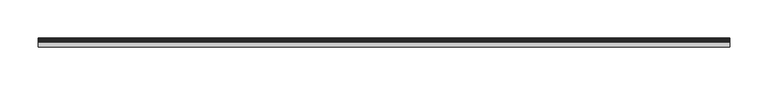
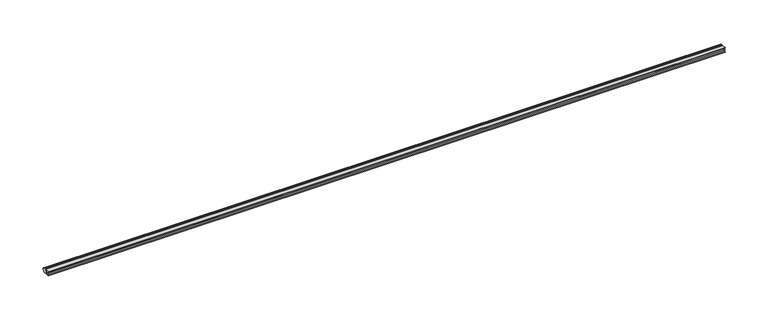
"""IFC4 building model written with IfcOpenShell, lengths in millimetres: proxy geometry, Generic Models 7:Generic Models 1:1:Generic Models 1:1 : Generic Models 7:Generic Models 1:337419:44 : Generic Models 7:Generic Models 1:1:Generic Models 1:1 : Generic Models 7:Generic Models 1:337419:306201."""

from ifc_helpers import new_model, si_unit, frame, origin, place, context, project, spatial, polyline, outline, extrude, source, transform, mapped, element, save


def generic_models_5b9f3622(model_context):
    return source(origin(), model_context, "Body", "SweptSolid", [
        extrude(outline(polyline([(-579079.4889203, 3909.2187499), (-579080.2717759, 3908.8672009), (-579081.4634893, 3907.8812291), (-579082.009811, 3906.6525036), (-579081.8252741, 3905.3732472), (-579080.9387475, 3904.2435877), (-579079.4889203, 3903.4402499), (-579084.8288841, 3903.4402499), (-579084.4854422, 3904.3190944), (-579084.1999879, 3906.3294999), (-579084.4854422, 3908.3399053), (-579084.8288841, 3909.2187499), (-579079.4889203, 3909.2187499)])), frame((592795.5032101, 0.0, 0.0), z_axis=(1.0, 0.0, 0.0), x_axis=(0.0, 1.0, 0.0)), (0.0, 0.0, 1.0), 910.0612812),
        extrude(outline(polyline([(-579076.3736413, 3909.1463103), (-579074.6358923, 3908.5884065), (-579073.4333327, 3907.5830985), (-579073.0041442, 3906.3294999), (-579073.4333327, 3905.0759013), (-579074.6358923, 3904.0705932), (-579076.3736413, 3903.5126894), (-579077.3380192, 3903.4402499), (-579078.3023971, 3903.5126894), (-579080.040146, 3904.0705932), (-579081.2427056, 3905.0759013), (-579081.6718942, 3906.3294999), (-579081.2427056, 3907.5830985), (-579080.040146, 3908.5884065), (-579078.3023971, 3909.1463103), (-579077.3380192, 3909.2187499), (-579076.3736413, 3909.1463103)])), frame((592795.5032101, 0.0, 0.0), z_axis=(1.0, 0.0, 0.0), x_axis=(0.0, 1.0, 0.0)), (0.0, 0.0, 1.0), 910.0612812),
    ])


if __name__ == "__main__":
    model = new_model("IFC4")
    model_context = context("Model", 3, world=origin())
    ifc_project = project(units=[si_unit("LENGTHUNIT", "METRE", prefix="MILLI")], contexts=[model_context])
    site = spatial("IfcSite", under=ifc_project)
    building = spatial("IfcBuilding", under=site)
    placement = place(None, origin())
    generic_models_shape = generic_models_5b9f3622(model_context)
    element("IfcBuildingElementProxy", 1, Name="Generic Models 7:Generic Models 1:1:Generic Models 1:1 : Generic Models 7:Generic Models 1:337419:44 : Generic Models 7:Generic Models 1:1:Generic Models 1:1 : Generic Models 7:Generic Models 1:337419:306201", ObjectType="Generic Models 7:Generic Models 1:1:Generic Models 1:1 : Generic Models 7:Generic Models 1:337419:44 : Generic Models 7:Generic Models 1:1:Generic Models 1:1 : Generic Models 7:Generic Models 1:337419:306201", at=placement, inside=building, context=model_context, shape_type="MappedRepresentation", body=[
        mapped(generic_models_shape, transform((0.0, 0.0, 0.0), x_axis=(1.0, 0.0, 0.0), y_axis=(0.0, 1.0, 0.0), z_axis=(0.0, 0.0, 1.0))),
    ])
    save(model, "model.ifc")

# Revit data of these elements
# Type "Generic Models 7:Generic Models 1:1:Generic Models 1:1 : Generic Models 7:Generic Models 1:337419:44 : Generic Models 7:Generic Models 1:1:Generic Models 1:1 : Generic Models 7:Generic Models 1:337419:306201"
#   NameOverride = "Generic Models 7:Generic Models 1:1:Generic Models 1:1 : Generic Models 7:Generic Models 1:337419:306201"
#   ObjectTypeOverride = "Generic Models 1:1 : Generic Models 7:Generic Models 1:337419"
#   Reference = "Generic Models 1"
#   Tag = "306201"
# Element 1 (IfcBuildingElementProxy, "Generic Models 7:Generic Models 1:1:Generic Models 1:1 : Generic Models 7:Generic Models 1:337419:44 : Generic Models 7:Generic Models 1:1:Generic Models 1:1 : Generic Models 7:Generic Models 1:337419:306201")
#   Materials on its faces: "SEMI-RIGID EPOXY SEALANT W/ BACKROD (REMOVE TEMP. JOINT FORM)"
# Materials
#   "SEMI-RIGID EPOXY SEALANT W/ BACKROD (REMOVE TEMP. JOINT FORM)": class "Unassigned", colour RGB 120 120 120, transparency 0, Cost = 0
